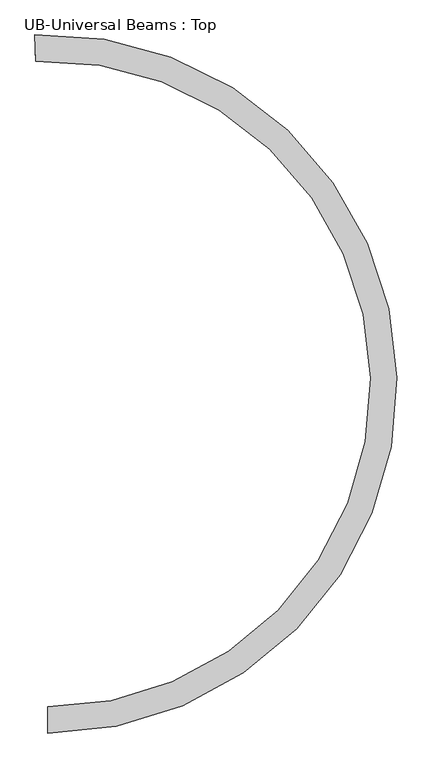
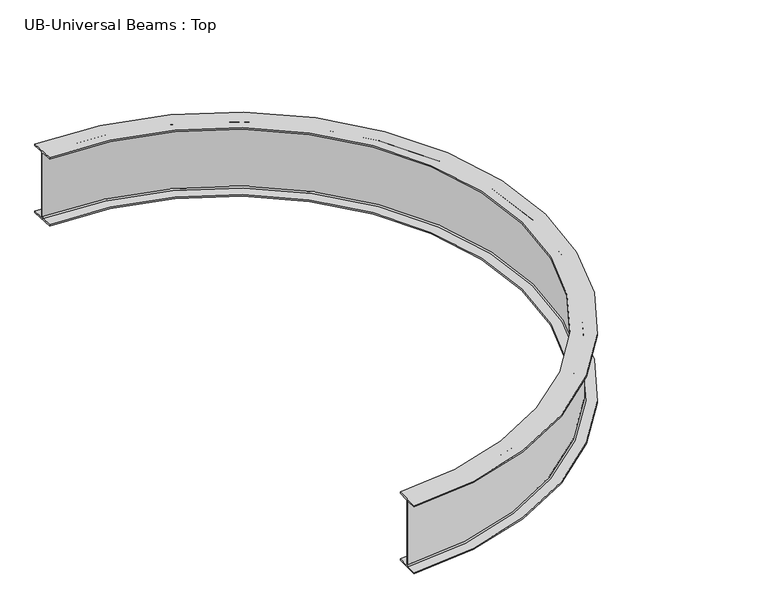
"""IFC4 building model written with IfcOpenShell, lengths in millimetres: beam geometry, UB-Universal Beams : Top."""

import ifcopenshell
import ifcopenshell.guid

model = None  # the IFC model being written
_history = None  # IfcOwnerHistory: only IFC2X3 demands one
_inside = {}  # id of a spatial element -> (the spatial element, [elements in it])
_under = {}  # id of a project, library or spatial element -> (it, [spatial elements below it])
_declared = {}  # id of a project -> (the project, [libraries it declares])
_typed = {}  # id of a type object -> (the type object, [elements of that type])
_made_of = {}  # id of a material, layer set ... -> (it, [elements and type objects made of it])


def new_model(schema):
    """Start an empty IFC model of exactly this schema.

    Asked for "IFC4X3", IfcOpenShell would pick the latest addendum, in which some entities
    have other attributes; the version numbers below select the first issue.
    IFC2X3 requires an IfcOwnerHistory on every rooted entity: one is made here for all.
    """
    global model, _history
    if schema == "IFC4X3":
        model = ifcopenshell.file(schema_version=(4, 3, 0, 0))
    else:
        model = ifcopenshell.file(schema=schema)
    _inside.clear()
    _under.clear()
    _declared.clear()
    _typed.clear()
    _made_of.clear()
    _history = None
    if model.schema == "IFC2X3":
        org = make("IfcOrganization", Name="unknown")
        user = make(
            "IfcPersonAndOrganization",
            ThePerson=make("IfcPerson", FamilyName="unknown"),
            TheOrganization=org,
        )
        app = make(
            "IfcApplication",
            ApplicationDeveloper=org,
            Version="unknown",
            ApplicationFullName="unknown",
            ApplicationIdentifier="unknown",
        )
        _history = make(
            "IfcOwnerHistory",
            OwningUser=user,
            OwningApplication=app,
            ChangeAction="ADDED",
            CreationDate=0,
        )
    return model


def make(cls, **values):
    """One entity of the class cls with the attributes given. An attribute that is None is left unset."""
    return model.create_entity(
        cls, **{name: value for name, value in values.items() if value is not None}
    )


def rooted(cls, **values):
    """An entity with a GlobalId (a new one), such as an element, a storey or a relation."""
    return make(cls, GlobalId=ifcopenshell.guid.new(), OwnerHistory=_history, **values)


def si_unit(unit_type, name, prefix=None):
    """IfcSIUnit, for example si_unit("LENGTHUNIT", "METRE", prefix="MILLI")."""
    return make("IfcSIUnit", UnitType=unit_type, Prefix=prefix, Name=name)


def assignment(units):
    """IfcUnitAssignment: the units of a project."""
    return None if units is None else make("IfcUnitAssignment", Units=units)


def point(xyz):
    """IfcCartesianPoint."""
    return None if xyz is None else make("IfcCartesianPoint", Coordinates=xyz)


def direction(xyz):
    """IfcDirection."""
    return None if xyz is None else make("IfcDirection", DirectionRatios=xyz)


def frame(location, z_axis=None, x_axis=None):
    """IfcAxis2Placement3D, a coordinate frame: its origin and axes. An axis left out is left unset."""
    return make(
        "IfcAxis2Placement3D",
        Location=point(location),
        Axis=direction(z_axis),
        RefDirection=direction(x_axis),
    )


def origin():
    """The frame at (0, 0, 0) with its axes left unset."""
    return frame((0.0, 0.0, 0.0))


def place(relative_to, where):
    """IfcLocalPlacement: puts the frame where relative to a parent placement (None: the world)."""
    return make(
        "IfcLocalPlacement", PlacementRelTo=relative_to, RelativePlacement=where
    )


def context(
    kind, dimensions, precision=None, world=None, true_north=None, identifier=None
):
    """IfcGeometricRepresentationContext, for example the 3D "Model" context."""
    return make(
        "IfcGeometricRepresentationContext",
        ContextIdentifier=identifier,
        ContextType=kind,
        CoordinateSpaceDimension=dimensions,
        Precision=precision,
        WorldCoordinateSystem=world,
        TrueNorth=true_north,
    )


def project(units=None, contexts=None):
    """IfcProject with its units and contexts."""
    return rooted(
        "IfcProject",
        Name="project",
        RepresentationContexts=contexts,
        UnitsInContext=assignment(units),
    )


def spatial(cls, under=None, at=None, **own):
    """A site, building, storey or space (cls), placed at a placement, below another one or the project."""
    s = rooted(cls, ObjectPlacement=at, **own)
    if under is not None:
        _under.setdefault(under.id(), (under, []))[1].append(s)
    return s


def polyline(points):
    """IfcPolyline through the points."""
    return make("IfcPolyline", Points=[point(p) for p in points])


def circle_curve(where, radius):
    """IfcCircle in the frame where."""
    return make("IfcCircle", Position=where, Radius=radius)


def ellipse_curve(where, semi_axis1, semi_axis2):
    """IfcEllipse in the frame where."""
    return make(
        "IfcEllipse", Position=where, SemiAxis1=semi_axis1, SemiAxis2=semi_axis2
    )


def trimmed(basis, trim1, trim2, sense, master):
    """IfcTrimmedCurve: the piece of a basis curve between two trims."""
    return make(
        "IfcTrimmedCurve",
        BasisCurve=basis,
        Trim1=trim1,
        Trim2=trim2,
        SenseAgreement=sense,
        MasterRepresentation=master,
    )


def shape(context_of_items, identifier, shape_type, items):
    """IfcShapeRepresentation: the items that make up one representation, for example the "Body"."""
    return make(
        "IfcShapeRepresentation",
        ContextOfItems=context_of_items,
        RepresentationIdentifier=identifier,
        RepresentationType=shape_type,
        Items=items,
    )


def source(mapping_origin, context_of_items, identifier, shape_type, items):
    """IfcRepresentationMap: a shape defined once, which mapped items show again and again."""
    return make(
        "IfcRepresentationMap",
        MappingOrigin=mapping_origin,
        MappedRepresentation=shape(context_of_items, identifier, shape_type, items),
    )


def transform(
    local_origin,
    x_axis=None,
    y_axis=None,
    z_axis=None,
    scale=None,
    scale2=None,
    scale3=None,
    uniform=True,
):
    """IfcCartesianTransformationOperator3D, or its non-uniform kind. x_axis, y_axis, z_axis: its Axis1, 2, 3."""
    if uniform:
        return make(
            "IfcCartesianTransformationOperator3D",
            Axis1=direction(x_axis),
            Axis2=direction(y_axis),
            LocalOrigin=point(local_origin),
            Scale=scale,
            Axis3=direction(z_axis),
        )
    return make(
        "IfcCartesianTransformationOperator3DnonUniform",
        Axis1=direction(x_axis),
        Axis2=direction(y_axis),
        LocalOrigin=point(local_origin),
        Scale=scale,
        Axis3=direction(z_axis),
        Scale2=scale2,
        Scale3=scale3,
    )


def mapped(mapping_source, mapping_target):
    """IfcMappedItem: shows the shape of a source again, moved by a transform."""
    return make(
        "IfcMappedItem", MappingSource=mapping_source, MappingTarget=mapping_target
    )


def made_of(thing, what):
    """Note that an element or type object is made of a material, layer set ...; save() writes the relation."""
    if what is not None:
        _made_of.setdefault(what.id(), (what, []))[1].append(thing)
    return thing


def element(
    cls,
    number,
    at=None,
    inside=None,
    cuts=None,
    type_object=None,
    material=None,
    context=None,
    identifier="Body",
    shape_type=None,
    held_by="IfcProductDefinitionShape",
    body=None,
    shapes=None,
    **own,
):
    """One element of the class cls, such as IfcWall. Its Tag is "e" and its number.

    at: its placement. inside: the storey or other place that contains it. cuts: it is an
    opening in that element (IfcRelVoidsElement). A single representation is given by context,
    identifier, shape_type and body (its items); several are given by shapes. held_by: the class
    of the entity that holds the representations. save() writes the other relations.
    """
    e = rooted(cls, Tag="e%d" % number, ObjectPlacement=at, **own)
    if body is not None:
        shapes = [shape(context, identifier, shape_type, body)]
    if shapes is not None:
        e.Representation = make(held_by, Representations=shapes)
    if inside is not None:
        _inside.setdefault(inside.id(), (inside, []))[1].append(e)
    if cuts is not None:
        rooted(
            "IfcRelVoidsElement", RelatingBuildingElement=cuts, RelatedOpeningElement=e
        )
    if type_object is not None:
        _typed.setdefault(type_object.id(), (type_object, []))[1].append(e)
    return made_of(e, material)


def aggregate(whole, parts):
    """IfcRelAggregates: a whole, such as a stair, and the parts it consists of."""
    return rooted("IfcRelAggregates", RelatingObject=whole, RelatedObjects=parts)


def save(model, path):
    """Write the relations noted so far, then the file.

    IfcRelAggregates (storeys below a building ...), IfcRelContainedInSpatialStructure (elements
    in a storey), IfcRelDefinesByType, IfcRelAssociatesMaterial and IfcRelDeclares: one each for
    every whole, place, type object, material and project.
    """
    for whole, parts in _under.values():
        aggregate(whole, parts)
    for where, things in _inside.values():
        rooted(
            "IfcRelContainedInSpatialStructure",
            RelatedElements=things,
            RelatingStructure=where,
        )
    for kind, things in _typed.values():
        rooted("IfcRelDefinesByType", RelatedObjects=things, RelatingType=kind)
    for what, things in _made_of.values():
        rooted("IfcRelAssociatesMaterial", RelatedObjects=things, RelatingMaterial=what)
    for by, libraries in _declared.values():
        rooted("IfcRelDeclares", RelatingContext=by, RelatedDefinitions=libraries)
    model.write(path)


def plane_surface(at):
    """IfcPlane: the flat surface through the origin of the frame at, square to its z axis."""
    return make("IfcPlane", Position=at)


def cylinder_surface(at, radius):
    """IfcCylindricalSurface: all points at the distance radius from the z axis of the frame at."""
    return make("IfcCylindricalSurface", Position=at, Radius=radius)


def revolved_surface(curve, axis_point, axis_direction):
    """IfcSurfaceOfRevolution: the curve turned about the line through axis_point along axis_direction."""
    return make(
        "IfcSurfaceOfRevolution",
        SweptCurve=make("IfcArbitraryOpenProfileDef", ProfileType="CURVE", Curve=curve),
        AxisPosition=make("IfcAxis1Placement", Location=point(axis_point), Axis=direction(axis_direction)),
    )


def advanced_brep(points, edges, surfaces, faces):
    """IfcAdvancedBrep: a solid bounded by faces that lie on surfaces and meet in shared edges.

    An edge is (start, end): straight between two places in points (the first is 0);
    or (start, end, curve); or (start, end, curve, False) where it runs against its curve.
    A face is (place in surfaces, loops), or (place, loops, False) where it looks against
    its surface's normal. A loop lists edges by number (the first is 1), with a minus sign
    where the edge is run from its end to its start. The first loop is the outer one.
    """
    corners = [point(p) for p in points]
    vertices = [make("IfcVertexPoint", VertexGeometry=c) for c in corners]
    made = []
    for start, end, *more in edges:
        made.append(
            make(
                "IfcEdgeCurve",
                EdgeStart=vertices[start],
                EdgeEnd=vertices[end],
                EdgeGeometry=more[0] if more else make("IfcPolyline", Points=[corners[start], corners[end]]),
                SameSense=more[1] if len(more) > 1 else True,
            )
        )
    hull = []
    for where, loops, *sense in faces:
        bounds = []
        for j, loop in enumerate(loops):
            ring = [make("IfcOrientedEdge", EdgeElement=made[abs(k) - 1], Orientation=k > 0) for k in loop]
            bounds.append(
                make(
                    "IfcFaceOuterBound" if j == 0 else "IfcFaceBound",
                    Bound=make("IfcEdgeLoop", EdgeList=ring),
                    Orientation=True,
                )
            )
        hull.append(make("IfcAdvancedFace", Bounds=bounds, FaceSurface=surfaces[where], SameSense=sense[0] if sense else True))
    return make("IfcAdvancedBrep", Outer=make("IfcClosedShell", CfsFaces=hull))


def ub_universal_beams_top_08d6708f(model_context):
    return source(origin(), model_context, "Body", "AdvancedBrep", [
        advanced_brep(
        [(-73.6052305, 4158.8116106, -239.8), (-76.1540227, 4229.3655875, -239.8), (-76.4753293, 4238.2597858, -230.9), (-76.4753293, 4238.2597858, 230.9), (-76.1540227, 4229.3655875, 239.8), (-73.6052305, 4158.8116106, 239.8), (-73.6052305, 4158.8116106, 250.0), (-79.5620394, 4323.7040496, 250.0), (-79.5620394, 4323.7040496, 239.8), (-77.0132472, 4253.1500727, 239.8), (-76.6919406, 4244.2558744, 230.9), (-76.6919406, 4244.2558744, -230.9), (-77.0132472, 4253.1500727, -239.8), (-79.5620394, 4323.7040496, -239.8), (-79.5620394, 4323.7040496, -250.0), (-73.6052305, 4158.8116106, -250.0), (0.0, 82.5, -239.8), (0.0, 82.5, -250.0), (0.0, -82.5, -250.0), (0.0, -82.5, -239.8), (0.0, -11.9, -239.8), (0.0, -3.0, -230.9), (0.0, -3.0, 230.9), (0.0, -11.9, 239.8), (0.0, -82.5, 239.8), (0.0, -82.5, 250.0), (0.0, 82.5, 250.0), (0.0, 82.5, 239.8), (0.0, 11.9, 239.8), (0.0, 3.0, 230.9), (0.0, 3.0, -230.9), (0.0, 11.9, -239.8)],
        [
            (0, 1),
            (1, 2, circle_curve(frame((-76.1540227, 4229.3655875, -230.9), z_axis=(0.9993481149514881, 0.03610187173689509, 0.0), x_axis=(-0.03610187173689509, 0.9993481149514881, 0.0)), 8.9)),
            (2, 3),
            (3, 4, circle_curve(frame((-76.1540227, 4229.3655875, 230.9), z_axis=(0.9993481149514881, 0.03610187173689509, 0.0), x_axis=(-0.03610187173689509, 0.9993481149514881, 0.0)), 8.9)),
            (4, 5),
            (5, 6),
            (6, 7),
            (7, 8),
            (8, 9),
            (9, 10, circle_curve(frame((-77.0132472, 4253.1500727, 230.9), z_axis=(0.9993481149514881, 0.03610187173689509, 0.0), x_axis=(-0.03610187173689509, 0.9993481149514881, 0.0)), 8.9)),
            (10, 11),
            (11, 12, circle_curve(frame((-77.0132472, 4253.1500727, -230.9), z_axis=(0.9993481149514881, 0.03610187173689509, 0.0), x_axis=(-0.03610187173689509, 0.9993481149514881, 0.0)), 8.9)),
            (12, 13),
            (13, 14),
            (14, 15),
            (15, 0),
            (16, 17),
            (17, 18),
            (18, 19),
            (19, 20),
            (20, 21, circle_curve(frame((0.0, -11.9, -230.9), z_axis=(1.0, 0.0, 0.0), x_axis=(0.0, -1.0, 0.0)), 8.9)),
            (21, 22),
            (22, 23, circle_curve(frame((0.0, -11.9, 230.9), z_axis=(1.0, 0.0, 0.0), x_axis=(0.0, -1.0, 0.0)), 8.9)),
            (23, 24),
            (24, 25),
            (25, 26),
            (26, 27),
            (27, 28),
            (28, 29, circle_curve(frame((0.0, 11.9, 230.9), z_axis=(1.0, 0.0, 0.0), x_axis=(0.0, -1.0, 0.0)), 8.9)),
            (29, 30),
            (30, 31, circle_curve(frame((0.0, 11.9, -230.9), z_axis=(1.0, 0.0, 0.0), x_axis=(0.0, -1.0, 0.0)), 8.9)),
            (31, 16),
            (0, 16, circle_curve(frame((0.0, 2121.3203436, -239.8), z_axis=(0.0, 0.0, -1.0), x_axis=(0.0, -1.0, 0.0)), 2038.8203436)),
            (31, 1, circle_curve(frame((0.0, 2121.3203436, -239.8), z_axis=(0.0, 0.0, 1.0), x_axis=(0.0, -1.0, 0.0)), 2109.4203436)),
            (30, 2, circle_curve(frame((0.0, 2121.3203436, -230.9), z_axis=(0.0, 0.0, 1.0), x_axis=(0.0, -1.0, 0.0)), 2118.3203436)),
            (29, 3, circle_curve(frame((0.0, 2121.3203436, 230.9), z_axis=(0.0, 0.0, 1.0), x_axis=(0.0, -1.0, 0.0)), 2118.3203436)),
            (28, 4, circle_curve(frame((0.0, 2121.3203436, 239.8), z_axis=(0.0, 0.0, 1.0), x_axis=(0.0, -1.0, 0.0)), 2109.4203436)),
            (27, 5, circle_curve(frame((0.0, 2121.3203436, 239.8), z_axis=(0.0, 0.0, 1.0), x_axis=(0.0, -1.0, 0.0)), 2038.8203436)),
            (26, 6, circle_curve(frame((0.0, 2121.3203436, 250.0), z_axis=(0.0, 0.0, 1.0), x_axis=(0.0, -1.0, 0.0)), 2038.8203436)),
            (25, 7, circle_curve(frame((0.0, 2121.3203436, 250.0), z_axis=(0.0, 0.0, 1.0), x_axis=(0.0, -1.0, 0.0)), 2203.8203436)),
            (24, 8, circle_curve(frame((0.0, 2121.3203436, 239.8), z_axis=(0.0, 0.0, 1.0), x_axis=(0.0, -1.0, 0.0)), 2203.8203436)),
            (23, 9, circle_curve(frame((0.0, 2121.3203436, 239.8), z_axis=(0.0, 0.0, 1.0), x_axis=(0.0, -1.0, 0.0)), 2133.2203436)),
            (22, 10, circle_curve(frame((0.0, 2121.3203436, 230.9), z_axis=(0.0, 0.0, 1.0), x_axis=(0.0, -1.0, 0.0)), 2124.3203436)),
            (21, 11, circle_curve(frame((0.0, 2121.3203436, -230.9), z_axis=(0.0, 0.0, 1.0), x_axis=(0.0, -1.0, 0.0)), 2124.3203436)),
            (20, 12, circle_curve(frame((0.0, 2121.3203436, -239.8), z_axis=(0.0, 0.0, 1.0), x_axis=(0.0, -1.0, 0.0)), 2133.2203436)),
            (19, 13, circle_curve(frame((0.0, 2121.3203436, -239.8), z_axis=(0.0, 0.0, 1.0), x_axis=(0.0, -1.0, 0.0)), 2203.8203436)),
            (18, 14, circle_curve(frame((0.0, 2121.3203436, -250.0), z_axis=(0.0, 0.0, 1.0), x_axis=(0.0, -1.0, 0.0)), 2203.8203436)),
            (17, 15, circle_curve(frame((0.0, 2121.3203436, -250.0), z_axis=(0.0, 0.0, 1.0), x_axis=(0.0, -1.0, 0.0)), 2038.8203436)),
        ],
        [
            plane_surface(frame((-76.583635, 4241.2578301, 0.0), z_axis=(-0.999348114951488, -0.03610187173690131, 0.0), x_axis=(0.0, 0.0, 1.0))),
            plane_surface(frame((0.0, 0.0, 0.0), z_axis=(-1.0, 0.0, 0.0), x_axis=(0.0, 0.0, 1.0))),
            plane_surface(frame((0.0, 2121.3203436, -239.8), z_axis=(0.0, 0.0, 1.0), x_axis=(0.0, -1.0, 0.0))),
            revolved_surface(trimmed(ellipse_curve(frame((0.0, 11.9, -230.9), z_axis=(1.0, 0.0, 0.0), x_axis=(0.0, -1.0, 0.0)), 8.9, 8.9), [point((0.0, 3.0, -230.9))], [point((0.0, 11.9, -239.8))], True, "CARTESIAN"), (0.0, 2121.3203436, 0.0), (0.0, 0.0, 1.0)),
            revolved_surface(polyline([(0.0, 3.0, 230.9), (0.0, 3.0, -230.9)]), (0.0, 2121.3203436, 0.0), (0.0, 0.0, 1.0)),
            revolved_surface(trimmed(ellipse_curve(frame((0.0, 11.9, 230.9), z_axis=(1.0, 0.0, 0.0), x_axis=(0.0, -1.0, 0.0)), 8.9, 8.9), [point((0.0, 11.9, 239.8))], [point((0.0, 3.0, 230.9))], True, "CARTESIAN"), (0.0, 2121.3203436, 0.0), (0.0, 0.0, 1.0)),
            plane_surface(frame((0.0, 2121.3203436, 239.8), z_axis=(0.0, 0.0, -1.0), x_axis=(0.0, -1.0, 0.0))),
            revolved_surface(polyline([(0.0, 82.5, 250.0), (0.0, 82.5, 239.8)]), (0.0, 2121.3203436, 0.0), (0.0, 0.0, 1.0)),
            plane_surface(frame((0.0, 2121.3203436, 250.0), z_axis=(0.0, 0.0, 1.0), x_axis=(0.0, -1.0, 0.0))),
            cylinder_surface(frame((0.0, 2121.3203436, 0.0), z_axis=(0.0, 0.0, 1.0), x_axis=(0.0, -1.0, 0.0)), 2203.8203436),
            revolved_surface(trimmed(ellipse_curve(frame((0.0, -11.9, 230.9), z_axis=(1.0, 0.0, 0.0), x_axis=(0.0, -1.0, 0.0)), 8.9, 8.9), [point((0.0, -3.0, 230.9))], [point((0.0, -11.9, 239.8))], True, "CARTESIAN"), (0.0, 2121.3203436, 0.0), (0.0, 0.0, 1.0)),
            cylinder_surface(frame((0.0, 2121.3203436, 0.0), z_axis=(0.0, 0.0, 1.0), x_axis=(0.0, -1.0, 0.0)), 2124.3203436),
            revolved_surface(trimmed(ellipse_curve(frame((0.0, -11.9, -230.9), z_axis=(1.0, 0.0, 0.0), x_axis=(0.0, -1.0, 0.0)), 8.9, 8.9), [point((0.0, -11.9, -239.8))], [point((0.0, -3.0, -230.9))], True, "CARTESIAN"), (0.0, 2121.3203436, 0.0), (0.0, 0.0, 1.0)),
            plane_surface(frame((0.0, 2121.3203436, -250.0), z_axis=(0.0, 0.0, -1.0), x_axis=(0.0, -1.0, 0.0))),
            revolved_surface(polyline([(0.0, 82.5, -239.8), (0.0, 82.5, -250.0)]), (0.0, 2121.3203436, 0.0), (0.0, 0.0, 1.0)),
        ],
        [
            (0, [[1, 2, 3, 4, 5, 6, 7, 8, 9, 10, 11, 12, 13, 14, 15, 16]]),
            (1, [[17, 18, 19, 20, 21, 22, 23, 24, 25, 26, 27, 28, 29, 30, 31, 32]]),
            (2, [[-1, 33, -32, 34]]),
            (3, [[-2, -34, -31, 35]]),
            (4, [[-3, -35, -30, 36]]),
            (5, [[-4, -36, -29, 37]]),
            (6, [[-5, -37, -28, 38]]),
            (7, [[-6, -38, -27, 39]]),
            (8, [[-7, -39, -26, 40]]),
            (9, [[-8, -40, -25, 41]]),
            (6, [[-9, -41, -24, 42]]),
            (10, [[-10, -42, -23, 43]]),
            (11, [[-11, -43, -22, 44]]),
            (12, [[-12, -44, -21, 45]]),
            (2, [[-13, -45, -20, 46]]),
            (9, [[-14, -46, -19, 47]]),
            (13, [[-15, -47, -18, 48]]),
            (14, [[-16, -48, -17, -33]]),
        ],
    ),
    ])


if __name__ == "__main__":
    model = new_model("IFC4")
    model_context = context("Model", 3, world=origin())
    ifc_project = project(units=[si_unit("LENGTHUNIT", "METRE", prefix="MILLI")], contexts=[model_context])
    site = spatial("IfcSite", under=ifc_project)
    building = spatial("IfcBuilding", under=site)
    placement = place(None, origin())
    ub_universal_beams_top_shape = ub_universal_beams_top_08d6708f(model_context)
    element("IfcBeam", 1, ObjectType="UB-Universal Beams : Top", at=placement, inside=building, context=model_context, shape_type="MappedRepresentation", body=[
        mapped(ub_universal_beams_top_shape, transform((0.0, 0.0, 0.0), x_axis=(1.0, 0.0, 0.0), y_axis=(0.0, 1.0, 0.0), z_axis=(0.0, 0.0, 1.0))),
    ])
    save(model, "model.ifc")

# Revit data of these elements
# Project information
#   Project Issue Date = "Issue Date"
#   Project Status = "Project Status"
#   Client Name = "Owner"
#   Project Address = "Enter address here"
#   Project Name = "Project Name"
#   Project Number = "Project Number"
# Type "UB-Universal Beams : Top"
#   Section Name Key = "UB305X165X40"
#   Width = 165 mm
#   Web Thickness = 6 mm
#   Web Fillet = 8.9 mm
#   Warping Constant = 164000 cm⁶
#   Torsional Moment of Inertia = 14.7 cm⁴
#   Section Area = 51.3 cm²
#   Plastic Modulus weak axis = 0.00501468 (stored number, unit not read)
#   Plastic Modulus strong axis = 0.022001 (stored number, unit not read)
#   Nominal Weight = 395.207 N/m
#   Moment of Inertia weak axis = 764 cm⁴
#   Moment of Inertia strong axis = 8503 cm⁴
#   Height = 500 mm
#   Flange Thickness = 10.2 mm
#   Elastic Modulus weak axis = 0.00327014 (stored number, unit not read)
#   Elastic Modulus strong axis = 0.0197762 (stored number, unit not read)
#   Centroid Vertical = 250 mm
#   Centroid Horizontal = 82.5 mm
#   Length [instance default] = 1500 mm
#   Structural Material [instance default] = Metal - Steel 43-275
#   Type Comments = ""
#   Assembly Code = ""
# Element 1 (IfcBeam, "UB-Universal Beams : Top")
#   Materials on its faces: "Metal - Steel 43-275"
# Materials
#   "Metal - Steel 43-275": class "Metal", colour RGB 247 247 247, transparency 0, Cost = 0
